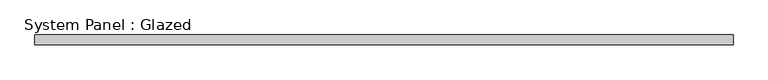
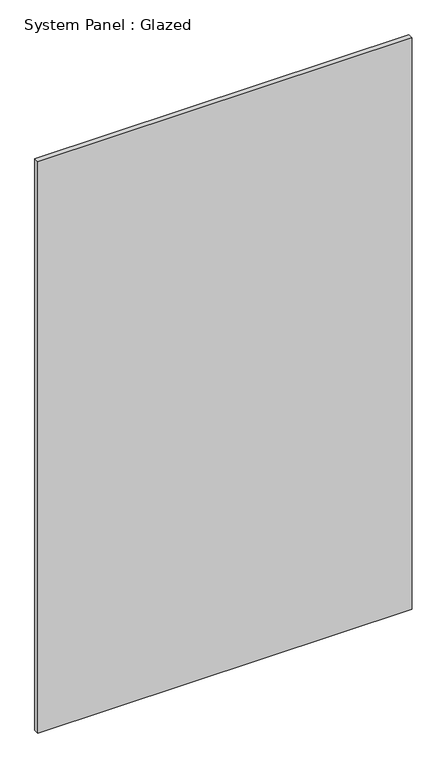
"""IFC4 building model written with IfcOpenShell, lengths in millimetres: plate geometry, System Panel : Glazed."""

from ifc_helpers import new_model, si_unit, origin, origin_with_axes, place, context, project, spatial, polyline, outline, extrude, source, transform, mapped, element, save


def system_panel_glazed_2ecdeac5(model_context):
    return source(origin(), model_context, "Body", "SweptSolid", [
        extrude(outline(polyline([(906.9444446, 24.5), (-906.9444446, 24.5), (-906.9444446, 49.5), (906.9444446, 49.5), (906.9444446, 24.5)])), origin_with_axes(), (0.0, 0.0, 1.0), 2925.0),
    ])


if __name__ == "__main__":
    model = new_model("IFC4")
    model_context = context("Model", 3, world=origin())
    ifc_project = project(units=[si_unit("LENGTHUNIT", "METRE", prefix="MILLI")], contexts=[model_context])
    site = spatial("IfcSite", under=ifc_project)
    building = spatial("IfcBuilding", under=site)
    placement = place(None, origin())
    system_panel_glazed_shape = system_panel_glazed_2ecdeac5(model_context)
    element("IfcPlate", 1, ObjectType="System Panel : Glazed", at=placement, inside=building, context=model_context, shape_type="MappedRepresentation", body=[
        mapped(system_panel_glazed_shape, transform((0.0, 0.0, 0.0), x_axis=(1.0, 0.0, 0.0), y_axis=(0.0, 1.0, 0.0), z_axis=(0.0, 0.0, 1.0))),
    ])
    save(model, "model.ifc")

# Revit data of these elements
# Element 1 (IfcPlate, "System Panel : Glazed")
#   Materials on its faces: "Glass"
# Materials
#   "Glass": class "Glass", colour RGB 0 128 192, transparency 0.9
